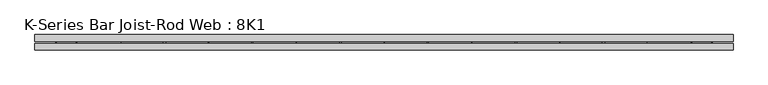
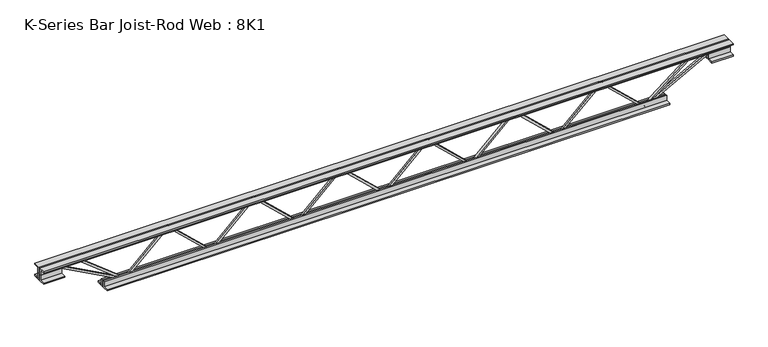
"""IFC4 building model written with IfcOpenShell, lengths in millimetres: beam geometry, K-Series Bar Joist-Rod Web : 8K1."""

from ifc_helpers import new_model, si_unit, frame, origin, place, context, project, spatial, polyline, outline, extrude, source, transform, mapped, element, save


def k_series_bar_joist_rod_web_8k1_170a1346(model_context):
    return source(origin(), model_context, "Body", "SweptSolid", [
        extrude(outline(polyline([(-90.4875, 416.1530704), (-100.0125, 416.1530704), (-100.0125, 421.2213977), (90.4875, 622.9479329), (90.4875, 625.5112783), (-100.0125, 827.2378135), (-100.0125, 832.3061408), (-90.4875, 832.3061408), (-90.4875, 831.0244681), (100.0125, 629.2979329), (100.0125, 619.1612783), (-90.4875, 417.4347431), (-90.4875, 416.1530704)])), frame((0.0, -4.7625, 0.0), z_axis=(0.0, 1.0, 0.0), x_axis=(0.0, 0.0, 1.0)), (0.0, 0.0, 1.0), 9.525),
        extrude(outline(polyline([(-90.4875, 0.0), (-100.0125, 0.0), (-100.0125, 5.0683273), (90.4875, 206.7948625), (90.4875, 209.3582079), (-100.0125, 411.0847431), (-100.0125, 416.1530704), (-90.4875, 416.1530704), (-90.4875, 414.8713977), (100.0125, 213.1448625), (100.0125, 203.0082079), (-90.4875, 1.2816727), (-90.4875, 0.0)])), frame((0.0, -4.7625, 0.0), z_axis=(0.0, 1.0, 0.0), x_axis=(0.0, 0.0, 1.0)), (0.0, 0.0, 1.0), 9.525),
        extrude(outline(polyline([(-90.4875, -416.1530704), (-100.0125, -416.1530704), (-100.0125, -411.0847431), (90.4875, -209.3582079), (90.4875, -206.7948625), (-100.0125, -5.0683273), (-100.0125, 0.0), (-90.4875, 0.0), (-90.4875, -1.2816727), (100.0125, -203.0082079), (100.0125, -213.1448625), (-90.4875, -414.8713977), (-90.4875, -416.1530704)])), frame((0.0, -4.7625, 0.0), z_axis=(0.0, 1.0, 0.0), x_axis=(0.0, 0.0, 1.0)), (0.0, 0.0, 1.0), 9.525),
        extrude(outline(polyline([(-90.4875, -832.3061408), (-100.0125, -832.3061408), (-100.0125, -827.2378135), (90.4875, -625.5112783), (90.4875, -622.9479329), (-100.0125, -421.2213977), (-100.0125, -416.1530704), (-90.4875, -416.1530704), (-90.4875, -417.4347431), (100.0125, -619.1612783), (100.0125, -629.2979329), (-90.4875, -831.0244681), (-90.4875, -832.3061408)])), frame((0.0, -4.7625, 0.0), z_axis=(0.0, 1.0, 0.0), x_axis=(0.0, 0.0, 1.0)), (0.0, 0.0, 1.0), 9.525),
        extrude(outline(polyline([(-90.4875, 832.3061408), (-100.0125, 832.3061408), (-100.0125, 837.3744681), (90.4875, 1039.1010033), (90.4875, 1041.6643486), (-100.0125, 1243.3908838), (-100.0125, 1248.4592111), (-90.4875, 1248.4592111), (-90.4875, 1247.1775385), (100.0125, 1045.4510033), (100.0125, 1035.3143486), (-90.4875, 833.5878135), (-90.4875, 832.3061408)])), frame((0.0, -4.7625, 0.0), z_axis=(0.0, 1.0, 0.0), x_axis=(0.0, 0.0, 1.0)), (0.0, 0.0, 1.0), 9.525),
        extrude(outline(polyline([(-90.4875, -1248.4592111), (-100.0125, -1248.4592111), (-100.0125, -1243.3908838), (90.4875, -1041.6643486), (90.4875, -1039.1010033), (-100.0125, -837.3744681), (-100.0125, -832.3061408), (-90.4875, -832.3061408), (-90.4875, -833.5878135), (100.0125, -1035.3143486), (100.0125, -1045.4510033), (-90.4875, -1247.1775385), (-90.4875, -1248.4592111)])), frame((0.0, -4.7625, 0.0), z_axis=(0.0, 1.0, 0.0), x_axis=(0.0, 0.0, 1.0)), (0.0, 0.0, 1.0), 9.525),
        extrude(outline(polyline([(4.7625, 101.6), (36.5125, 101.6), (36.5125, 95.25), (11.1125, 95.25), (11.1125, 69.85), (4.7625, 69.85), (4.7625, 101.6)])), frame((-1654.8592111, 0.0, 0.0), z_axis=(1.0, 0.0, 0.0), x_axis=(0.0, 1.0, 0.0)), (0.0, 0.0, 1.0), 3309.7184223),
        extrude(outline(polyline([(-4.7625, 101.6), (-4.7625, 69.85), (-11.1125, 69.85), (-11.1125, 95.25), (-36.5125, 95.25), (-36.5125, 101.6), (-4.7625, 101.6)])), frame((-1654.8592111, 0.0, 0.0), z_axis=(1.0, 0.0, 0.0), x_axis=(0.0, 1.0, 0.0)), (0.0, 0.0, 1.0), 3309.7184223),
        extrude(outline(polyline([(-4.7625, 38.1), (-36.5125, 38.1), (-36.5125, 44.45), (-11.1125, 44.45), (-11.1125, 69.85), (-4.7625, 69.85), (-4.7625, 38.1)])), frame((-1654.8592111, 0.0, 0.0), z_axis=(1.0, 0.0, 0.0), x_axis=(0.0, 1.0, 0.0)), (0.0, 0.0, 1.0), 101.6),
        extrude(outline(polyline([(36.5125, 38.1), (4.7625, 38.1), (4.7625, 69.85), (11.1125, 69.85), (11.1125, 44.45), (36.5125, 44.45), (36.5125, 38.1)])), frame((-1654.8592111, 0.0, 0.0), z_axis=(1.0, 0.0, 0.0), x_axis=(0.0, 1.0, 0.0)), (0.0, 0.0, 1.0), 101.6),
        extrude(outline(polyline([(4.7625, 38.1), (4.7625, 69.85), (11.1125, 69.85), (11.1125, 44.45), (36.5125, 44.45), (36.5125, 38.1), (4.7625, 38.1)])), frame((1553.2592111, 0.0, 0.0), z_axis=(1.0, 0.0, 0.0), x_axis=(0.0, 1.0, 0.0)), (0.0, 0.0, 1.0), 101.6),
        extrude(outline(polyline([(-4.7625, 38.1), (-36.5125, 38.1), (-36.5125, 44.45), (-11.1125, 44.45), (-11.1125, 69.85), (-4.7625, 69.85), (-4.7625, 38.1)])), frame((1553.2592111, 0.0, 0.0), z_axis=(1.0, 0.0, 0.0), x_axis=(0.0, 1.0, 0.0)), (0.0, 0.0, 1.0), 101.6),
        extrude(outline(polyline([(4.7625, -101.6), (4.7625, -69.85), (11.1125, -69.85), (11.1125, -95.25), (36.5125, -95.25), (36.5125, -101.6), (4.7625, -101.6)])), frame((-1350.0592111, 0.0, 0.0), z_axis=(1.0, 0.0, 0.0), x_axis=(0.0, 1.0, 0.0)), (0.0, 0.0, 1.0), 2700.1184223),
        extrude(outline(polyline([(-4.7625, -101.6), (-36.5125, -101.6), (-36.5125, -95.25), (-11.1125, -95.25), (-11.1125, -69.85), (-4.7625, -69.85), (-4.7625, -101.6)])), frame((-1350.0592111, 0.0, 0.0), z_axis=(1.0, 0.0, 0.0), x_axis=(0.0, 1.0, 0.0)), (0.0, 0.0, 1.0), 2700.1184223),
        extrude(outline(polyline([(0.0, -9.525), (0.0, 0.0), (346.6425392, 0.0), (346.6425392, -9.525), (0.0, -9.525)])), frame((-1555.5275096, 4.7625, 65.662372), z_axis=(0.4762831485400794, 0.0, 0.8792919665371387), x_axis=(0.8792919665371387, 0.0, -0.4762831485400794)), (0.0, 0.0, 1.0), 9.525),
        extrude(outline(polyline([(0.0, -9.525), (0.0, 0.0), (265.6197555, 0.0), (265.6197555, -9.525), (0.0, -9.525)])), frame((-1459.4959507, 4.7625, 66.1192365), z_axis=(0.6215652134239323, 0.0, 0.7833624228039416), x_axis=(0.7833624228039416, 0.0, -0.6215652134239323)), (0.0, 0.0, 1.0), 9.525),
        extrude(outline(polyline([(0.0, -9.525), (0.0, 0.0), (346.6425392, 0.0), (346.6425392, -9.525), (0.0, -9.525)])), frame((1555.5275096, -4.7625, 65.662372), z_axis=(-0.4762831485400428, 0.0, 0.8792919665371586), x_axis=(-0.8792919665371586, 0.0, -0.4762831485400428)), (0.0, 0.0, 1.0), 9.525),
        extrude(outline(polyline([(0.0, -9.525), (0.0, 0.0), (265.6197555, 0.0), (265.6197555, -9.525), (0.0, -9.525)])), frame((1459.4959507, -4.7625, 66.1192365), z_axis=(-0.6215652134239079, 0.0, 0.7833624228039611), x_axis=(-0.7833624228039611, 0.0, -0.6215652134239079)), (0.0, 0.0, 1.0), 9.525),
    ])


if __name__ == "__main__":
    model = new_model("IFC4")
    model_context = context("Model", 3, world=origin())
    ifc_project = project(units=[si_unit("LENGTHUNIT", "METRE", prefix="MILLI")], contexts=[model_context])
    site = spatial("IfcSite", under=ifc_project)
    building = spatial("IfcBuilding", under=site)
    placement = place(None, origin())
    k_series_bar_joist_rod_web_8k1_shape = k_series_bar_joist_rod_web_8k1_170a1346(model_context)
    element("IfcBeam", 1, ObjectType="K-Series Bar Joist-Rod Web : 8K1", at=placement, inside=building, context=model_context, shape_type="MappedRepresentation", body=[
        mapped(k_series_bar_joist_rod_web_8k1_shape, transform((0.0, 0.0, 0.0), x_axis=(1.0, 0.0, 0.0), y_axis=(0.0, 1.0, 0.0), z_axis=(0.0, 0.0, 1.0))),
    ])
    save(model, "model.ifc")

# Revit data of these elements
# Type "K-Series Bar Joist-Rod Web : 8K1"
#   Assembly Code = "B1010350"
#   Wt = 5.1
#   Web Thickness = 0' - 0 3/8"
#   Start Offset [instance default] = 0' - 0"
#   Start Extension [instance default] = 0' - 0"
#   Seat Length = 0' - 4"
#   Seat Depth = 0' - 2 1/2"
#   PanelArrayLength [instance default] = 21' - 4"
#   Panel [instance default] = 1' - 4"
#   End Offset [instance default] = 0' - 0"
#   End Extension [instance default] = 0' - 0"
#   End Panel = 1' - 4"
#   Cord Leg = 0' - 1 1/4"
#   Chord Thickness = 0' - 0 1/4"
#   Length [instance default] = 24' - 0"
#   Depth = 0' - 8"
#   PanelArrayNum [instance default] = 16
#   Rendering Material = none
# Element 1 (IfcBeam, "K-Series Bar Joist-Rod Web : 8K1")
#   PanelArrayLength = 8' - 2.30387"
#   Panel = 1' - 4.38398"
#   PanelArrayNum = 6
